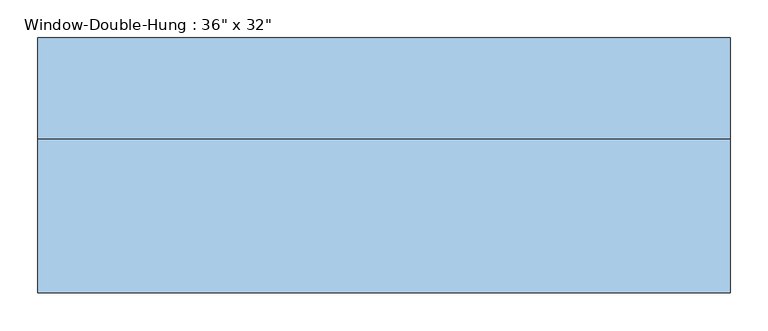
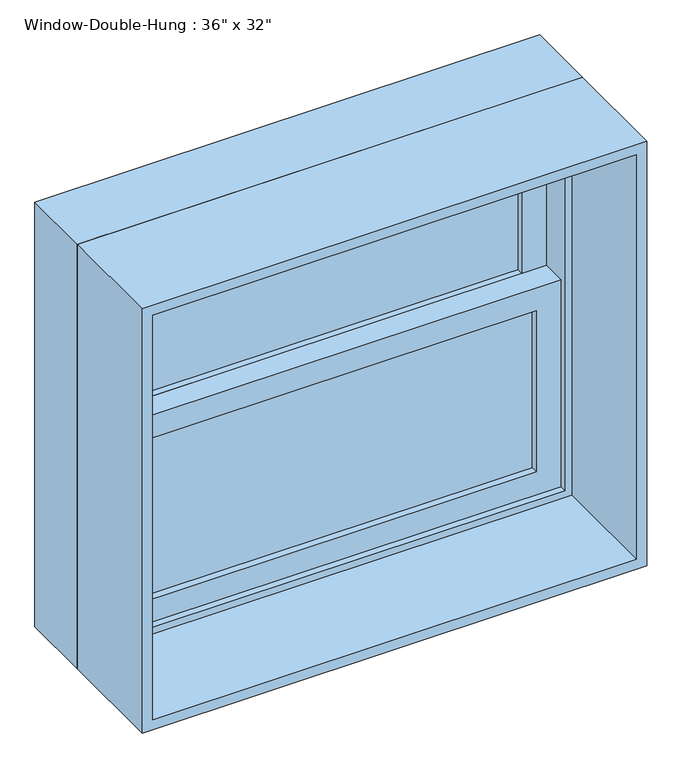
"""IFC4 building model written with IfcOpenShell, lengths in millimetres: window geometry."""

import ifcopenshell
import ifcopenshell.guid

model = None  # the IFC model being written
_history = None  # IfcOwnerHistory: only IFC2X3 demands one
_inside = {}  # id of a spatial element -> (the spatial element, [elements in it])
_under = {}  # id of a project, library or spatial element -> (it, [spatial elements below it])
_declared = {}  # id of a project -> (the project, [libraries it declares])
_typed = {}  # id of a type object -> (the type object, [elements of that type])
_made_of = {}  # id of a material, layer set ... -> (it, [elements and type objects made of it])


def new_model(schema):
    """Start an empty IFC model of exactly this schema.

    Asked for "IFC4X3", IfcOpenShell would pick the latest addendum, in which some entities
    have other attributes; the version numbers below select the first issue.
    IFC2X3 requires an IfcOwnerHistory on every rooted entity: one is made here for all.
    """
    global model, _history
    if schema == "IFC4X3":
        model = ifcopenshell.file(schema_version=(4, 3, 0, 0))
    else:
        model = ifcopenshell.file(schema=schema)
    _inside.clear()
    _under.clear()
    _declared.clear()
    _typed.clear()
    _made_of.clear()
    _history = None
    if model.schema == "IFC2X3":
        org = make("IfcOrganization", Name="unknown")
        user = make(
            "IfcPersonAndOrganization",
            ThePerson=make("IfcPerson", FamilyName="unknown"),
            TheOrganization=org,
        )
        app = make(
            "IfcApplication",
            ApplicationDeveloper=org,
            Version="unknown",
            ApplicationFullName="unknown",
            ApplicationIdentifier="unknown",
        )
        _history = make(
            "IfcOwnerHistory",
            OwningUser=user,
            OwningApplication=app,
            ChangeAction="ADDED",
            CreationDate=0,
        )
    return model


def make(cls, **values):
    """One entity of the class cls with the attributes given. An attribute that is None is left unset."""
    return model.create_entity(
        cls, **{name: value for name, value in values.items() if value is not None}
    )


def rooted(cls, **values):
    """An entity with a GlobalId (a new one), such as an element, a storey or a relation."""
    return make(cls, GlobalId=ifcopenshell.guid.new(), OwnerHistory=_history, **values)


def si_unit(unit_type, name, prefix=None):
    """IfcSIUnit, for example si_unit("LENGTHUNIT", "METRE", prefix="MILLI")."""
    return make("IfcSIUnit", UnitType=unit_type, Prefix=prefix, Name=name)


def assignment(units):
    """IfcUnitAssignment: the units of a project."""
    return None if units is None else make("IfcUnitAssignment", Units=units)


def point(xyz):
    """IfcCartesianPoint."""
    return None if xyz is None else make("IfcCartesianPoint", Coordinates=xyz)


def direction(xyz):
    """IfcDirection."""
    return None if xyz is None else make("IfcDirection", DirectionRatios=xyz)


def frame(location, z_axis=None, x_axis=None):
    """IfcAxis2Placement3D, a coordinate frame: its origin and axes. An axis left out is left unset."""
    return make(
        "IfcAxis2Placement3D",
        Location=point(location),
        Axis=direction(z_axis),
        RefDirection=direction(x_axis),
    )


def origin():
    """The frame at (0, 0, 0) with its axes left unset."""
    return frame((0.0, 0.0, 0.0))


def place(relative_to, where):
    """IfcLocalPlacement: puts the frame where relative to a parent placement (None: the world)."""
    return make(
        "IfcLocalPlacement", PlacementRelTo=relative_to, RelativePlacement=where
    )


def context(
    kind, dimensions, precision=None, world=None, true_north=None, identifier=None
):
    """IfcGeometricRepresentationContext, for example the 3D "Model" context."""
    return make(
        "IfcGeometricRepresentationContext",
        ContextIdentifier=identifier,
        ContextType=kind,
        CoordinateSpaceDimension=dimensions,
        Precision=precision,
        WorldCoordinateSystem=world,
        TrueNorth=true_north,
    )


def project(units=None, contexts=None):
    """IfcProject with its units and contexts."""
    return rooted(
        "IfcProject",
        Name="project",
        RepresentationContexts=contexts,
        UnitsInContext=assignment(units),
    )


def spatial(cls, under=None, at=None, **own):
    """A site, building, storey or space (cls), placed at a placement, below another one or the project."""
    s = rooted(cls, ObjectPlacement=at, **own)
    if under is not None:
        _under.setdefault(under.id(), (under, []))[1].append(s)
    return s


def polyline(points):
    """IfcPolyline through the points."""
    return make("IfcPolyline", Points=[point(p) for p in points])


def outline(outer, holes=None, kind="AREA"):
    """IfcArbitraryClosedProfileDef: a profile drawn as a closed curve; with holes, ...WithVoids."""
    if holes is None:
        return make("IfcArbitraryClosedProfileDef", ProfileType=kind, OuterCurve=outer)
    return make(
        "IfcArbitraryProfileDefWithVoids",
        ProfileType=kind,
        OuterCurve=outer,
        InnerCurves=holes,
    )


def extrude(swept, where, along, depth):
    """IfcExtrudedAreaSolid: the profile swept, set in the frame where, extruded along a direction by depth."""
    return make(
        "IfcExtrudedAreaSolid",
        SweptArea=swept,
        Position=where,
        ExtrudedDirection=direction(along),
        Depth=depth,
    )


def shape(context_of_items, identifier, shape_type, items):
    """IfcShapeRepresentation: the items that make up one representation, for example the "Body"."""
    return make(
        "IfcShapeRepresentation",
        ContextOfItems=context_of_items,
        RepresentationIdentifier=identifier,
        RepresentationType=shape_type,
        Items=items,
    )


def source(mapping_origin, context_of_items, identifier, shape_type, items):
    """IfcRepresentationMap: a shape defined once, which mapped items show again and again."""
    return make(
        "IfcRepresentationMap",
        MappingOrigin=mapping_origin,
        MappedRepresentation=shape(context_of_items, identifier, shape_type, items),
    )


def transform(
    local_origin,
    x_axis=None,
    y_axis=None,
    z_axis=None,
    scale=None,
    scale2=None,
    scale3=None,
    uniform=True,
):
    """IfcCartesianTransformationOperator3D, or its non-uniform kind. x_axis, y_axis, z_axis: its Axis1, 2, 3."""
    if uniform:
        return make(
            "IfcCartesianTransformationOperator3D",
            Axis1=direction(x_axis),
            Axis2=direction(y_axis),
            LocalOrigin=point(local_origin),
            Scale=scale,
            Axis3=direction(z_axis),
        )
    return make(
        "IfcCartesianTransformationOperator3DnonUniform",
        Axis1=direction(x_axis),
        Axis2=direction(y_axis),
        LocalOrigin=point(local_origin),
        Scale=scale,
        Axis3=direction(z_axis),
        Scale2=scale2,
        Scale3=scale3,
    )


def mapped(mapping_source, mapping_target):
    """IfcMappedItem: shows the shape of a source again, moved by a transform."""
    return make(
        "IfcMappedItem", MappingSource=mapping_source, MappingTarget=mapping_target
    )


def made_of(thing, what):
    """Note that an element or type object is made of a material, layer set ...; save() writes the relation."""
    if what is not None:
        _made_of.setdefault(what.id(), (what, []))[1].append(thing)
    return thing


def element(
    cls,
    number,
    at=None,
    inside=None,
    cuts=None,
    type_object=None,
    material=None,
    context=None,
    identifier="Body",
    shape_type=None,
    held_by="IfcProductDefinitionShape",
    body=None,
    shapes=None,
    **own,
):
    """One element of the class cls, such as IfcWall. Its Tag is "e" and its number.

    at: its placement. inside: the storey or other place that contains it. cuts: it is an
    opening in that element (IfcRelVoidsElement). A single representation is given by context,
    identifier, shape_type and body (its items); several are given by shapes. held_by: the class
    of the entity that holds the representations. save() writes the other relations.
    """
    e = rooted(cls, Tag="e%d" % number, ObjectPlacement=at, **own)
    if body is not None:
        shapes = [shape(context, identifier, shape_type, body)]
    if shapes is not None:
        e.Representation = make(held_by, Representations=shapes)
    if inside is not None:
        _inside.setdefault(inside.id(), (inside, []))[1].append(e)
    if cuts is not None:
        rooted(
            "IfcRelVoidsElement", RelatingBuildingElement=cuts, RelatedOpeningElement=e
        )
    if type_object is not None:
        _typed.setdefault(type_object.id(), (type_object, []))[1].append(e)
    return made_of(e, material)


def aggregate(whole, parts):
    """IfcRelAggregates: a whole, such as a stair, and the parts it consists of."""
    return rooted("IfcRelAggregates", RelatingObject=whole, RelatedObjects=parts)


def save(model, path):
    """Write the relations noted so far, then the file.

    IfcRelAggregates (storeys below a building ...), IfcRelContainedInSpatialStructure (elements
    in a storey), IfcRelDefinesByType, IfcRelAssociatesMaterial and IfcRelDeclares: one each for
    every whole, place, type object, material and project.
    """
    for whole, parts in _under.values():
        aggregate(whole, parts)
    for where, things in _inside.values():
        rooted(
            "IfcRelContainedInSpatialStructure",
            RelatedElements=things,
            RelatingStructure=where,
        )
    for kind, things in _typed.values():
        rooted("IfcRelDefinesByType", RelatedObjects=things, RelatingType=kind)
    for what, things in _made_of.values():
        rooted("IfcRelAssociatesMaterial", RelatedObjects=things, RelatingMaterial=what)
    for by, libraries in _declared.values():
        rooted("IfcRelDeclares", RelatingContext=by, RelatedDefinitions=libraries)
    model.write(path)


def window_21393ef8(model_context):
    return source(origin(), model_context, "Body", "SweptSolid", [
        extrude(outline(polyline([(381.0, 88.9), (381.0, 82.55), (-381.0, 82.55), (-381.0, 88.9), (381.0, 88.9)])), frame((0.0, 0.0, 990.6), z_axis=(0.0, 0.0, 1.0), x_axis=(1.0, 0.0, 0.0)), (0.0, 0.0, 1.0), 307.975),
        extrude(outline(polyline([(-381.0, 76.2), (381.0, 76.2), (381.0, 69.85), (-381.0, 69.85), (-381.0, 76.2)])), frame((0.0, 0.0, 990.6), z_axis=(0.0, 0.0, 1.0), x_axis=(1.0, 0.0, 0.0)), (0.0, 0.0, 1.0), 307.975),
        extrude(outline(polyline([(381.0, 133.35), (381.0, 127.0), (-381.0, 127.0), (-381.0, 133.35), (381.0, 133.35)])), frame((0.0, 0.0, 1343.025), z_axis=(0.0, 0.0, 1.0), x_axis=(1.0, 0.0, 0.0)), (0.0, 0.0, 1.0), 307.975),
        extrude(outline(polyline([(-381.0, 120.65), (381.0, 120.65), (381.0, 114.3), (-381.0, 114.3), (-381.0, 120.65)])), frame((0.0, 0.0, 1343.025), z_axis=(0.0, 0.0, 1.0), x_axis=(1.0, 0.0, 0.0)), (0.0, 0.0, 1.0), 307.975),
        extrude(outline(polyline([(1343.025, -425.45), (946.15, -425.45), (946.15, 425.45), (1343.025, 425.45), (1343.025, -425.45)]), holes=[polyline([(1298.575, 381.0), (990.6, 381.0), (990.6, -381.0), (1298.575, -381.0), (1298.575, 381.0)])]), frame((0.0, 57.15, 0.0), z_axis=(0.0, 1.0, 0.0), x_axis=(0.0, 0.0, 1.0)), (0.0, 0.0, 1.0), 44.45),
        extrude(outline(polyline([(1695.45, -425.45), (1298.575, -425.45), (1298.575, 425.45), (1695.45, 425.45), (1695.45, -425.45)]), holes=[polyline([(1651.0, 381.0), (1343.025, 381.0), (1343.025, -381.0), (1651.0, -381.0), (1651.0, 381.0)])]), frame((0.0, 101.6, 0.0), z_axis=(0.0, 1.0, 0.0), x_axis=(0.0, 0.0, 1.0)), (0.0, 0.0, 1.0), 44.45),
        extrude(outline(polyline([(1727.2, -457.2), (914.4, -457.2), (914.4, 457.2), (1727.2, 457.2), (1727.2, -457.2)]), holes=[polyline([(1695.45, 425.45), (946.15, 425.45), (946.15, -425.45), (1695.45, -425.45), (1695.45, 425.45)])]), frame((0.0, 44.45, 0.0), z_axis=(0.0, 1.0, 0.0), x_axis=(0.0, 0.0, 1.0)), (0.0, 0.0, 1.0), 133.35),
        extrude(outline(polyline([(1727.2, 457.2), (1727.2, -457.2), (914.4, -457.2), (914.4, 457.2), (1727.2, 457.2)]), holes=[polyline([(1708.15, 438.15), (933.45, 438.15), (933.45, -438.15), (1708.15, -438.15), (1708.15, 438.15)])]), frame((0.0, -158.75, 0.0), z_axis=(0.0, 1.0, 0.0), x_axis=(0.0, 0.0, 1.0)), (0.0, 0.0, 1.0), 203.2),
    ])


if __name__ == "__main__":
    model = new_model("IFC4")
    model_context = context("Model", 3, world=origin())
    ifc_project = project(units=[si_unit("LENGTHUNIT", "METRE", prefix="MILLI")], contexts=[model_context])
    site = spatial("IfcSite", under=ifc_project)
    building = spatial("IfcBuilding", under=site)
    placement = place(None, origin())
    window_shape = window_21393ef8(model_context)
    element("IfcWindow", 1, ObjectType="Window-Double-Hung : 36\" x 32\"", at=placement, inside=building, context=model_context, shape_type="MappedRepresentation", body=[
        mapped(window_shape, transform((0.0, 0.0, 0.0), x_axis=(1.0, 0.0, 0.0), y_axis=(0.0, 1.0, 0.0), z_axis=(0.0, 0.0, 1.0))),
    ])
    save(model, "model.ifc")

# Revit data of these elements
# Type "Window-Double-Hung : 36\" x 32\""
#   Type Mark = "19"
#   Fire Rating = "0.5h"
#   Construction Type Id = "DG-DR"
#   Assembly Code = "B2020100"
#   Analytic Construction = "Double glazing - domestic"
#   Wall Thickness [instance default] = 0' - 6"
#   Window Inset [instance default] = 0' - 0"
#   Visual Light Transmittance = 0.81
#   Thermal Resistance (R) = 1.8146 (h·ft²·°F)/BTU
#   Solar Heat Gain Coefficient = 0.76
#   Muntin Width = 2' - 6"
#   Muntin Height = 1' - 0 1/8"
#   Interior Wall Closure [instance default] = 0' - 1 1/2"
#   Rough Width = 3' - 0 1/2"
#   Rough Height = 2' - 8 1/2"
#   Frame Extension [instance default] = 0' - 1 1/4"
#   Exterior Wall Closure [instance default] = 0' - 0 1/2"
#   Extension Jamb [instance default] = 0' - 1 1/2"
#   Heat Transfer Coefficient (U) = 0.5511 BTU/(h·ft²·°F)
#   Height = 2' - 8"
#   Width = 3' - 0"
#   Top Muntin Visibility = yes
#   Indicator Visibility [instance default] = yes
#   Extension Jamb Visibility [instance default] = yes
#   Interior Trim Visibility [instance default] = yes
#   Exterior Trim Visibility [instance default] = yes
#   Define Thermal Properties by = 1
#   Bottom Muntin Visibility = yes
#   Muntin Pattern = Muntin Pattern_2x2 : Muntin Pattern_2x2
#   Interior Trim Material = Wood - Stained
#   Interior Trim = Trim-Window-Interior-Flat : Picture Frame
#   Exterior Trim Material = Clad - White
#   Exterior Trim = Trim-Window-Exterior-Flat : with Sill
#   Glass Panel Material = Glass
#   Exterior Frame Material = Clad - White
#   Interior Frame Material = Wood - Stained
#   Wall Closure = (empty or 0)
# Element 1 (IfcWindow, "Window-Double-Hung : 36\" x 32\"")
#   Wall Thickness = 1' - 0 1/2"
#   Extension Jamb = 0' - 8"
#   Materials on its faces: "Wood - Stained", "Glass", "Clad - White"
# Materials
#   "Wood - Stained": class "Wood", colour RGB 224 178 126, transparency 0, Cost = 0
#   "Clad - White": class "Wood", colour RGB 242 242 238, transparency 0, Cost = 0
#   "Glass": class "Glass", colour RGB 0 128 192, transparency 0.75, Description = "Soda Lime Glass", Cost = 0
